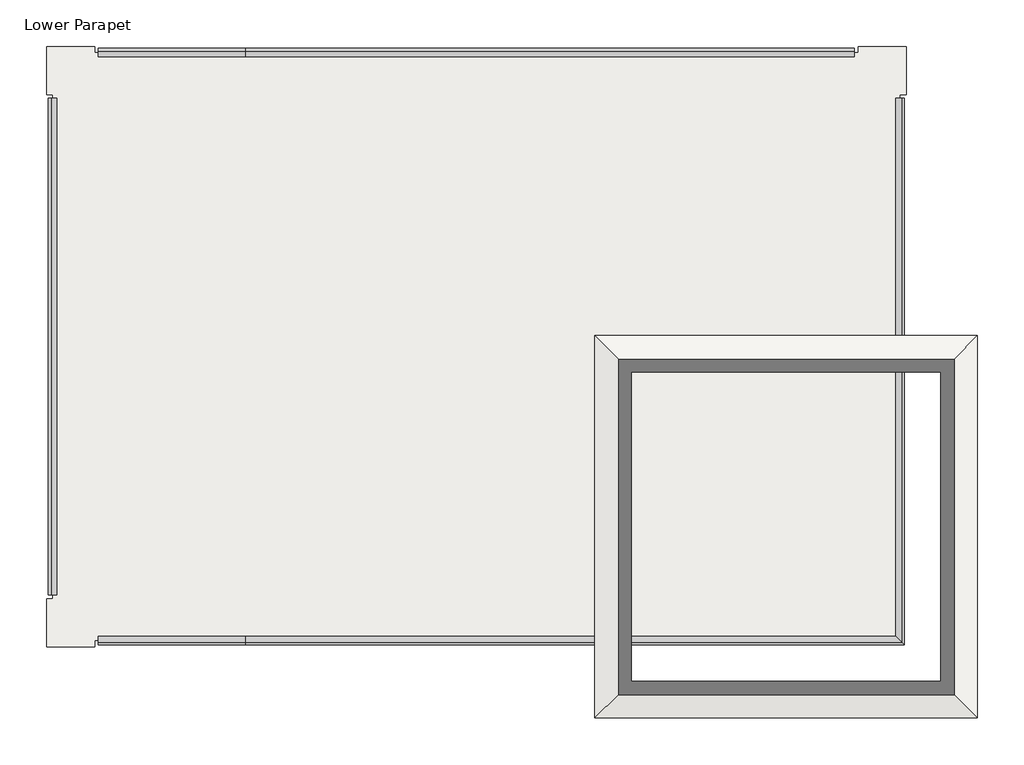
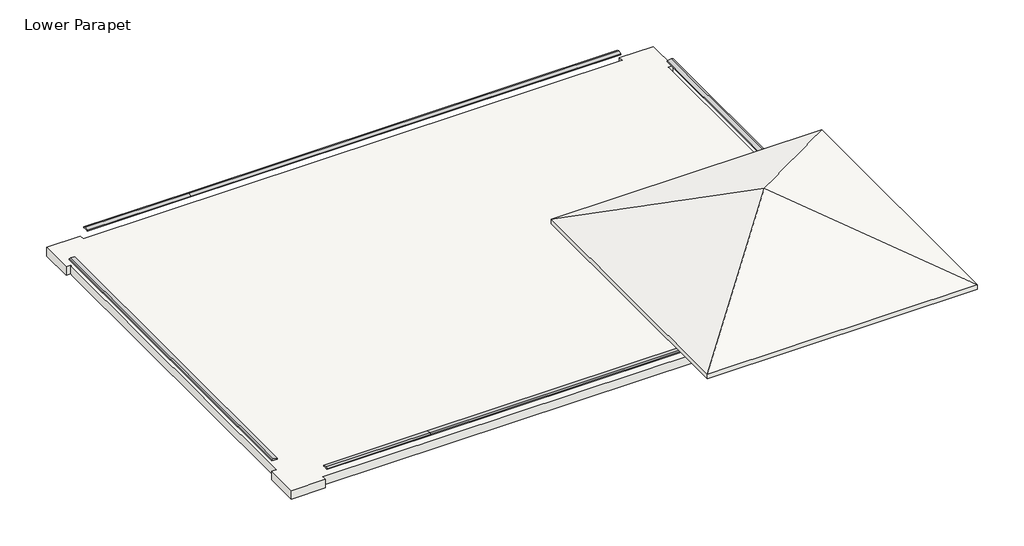
# One storey: 6 proxies, 2 roofs.
"""IFC4 building model written with IfcOpenShell, lengths in millimetres."""

import ifcopenshell
import ifcopenshell.guid

model = None  # the IFC model being written
_history = None  # IfcOwnerHistory: only IFC2X3 demands one
_inside = {}  # id of a spatial element -> (the spatial element, [elements in it])
_under = {}  # id of a project, library or spatial element -> (it, [spatial elements below it])
_declared = {}  # id of a project -> (the project, [libraries it declares])
_typed = {}  # id of a type object -> (the type object, [elements of that type])
_made_of = {}  # id of a material, layer set ... -> (it, [elements and type objects made of it])


def new_model(schema):
    """Start an empty IFC model of exactly this schema.

    Asked for "IFC4X3", IfcOpenShell would pick the latest addendum, in which some entities
    have other attributes; the version numbers below select the first issue.
    IFC2X3 requires an IfcOwnerHistory on every rooted entity: one is made here for all.
    """
    global model, _history
    if schema == "IFC4X3":
        model = ifcopenshell.file(schema_version=(4, 3, 0, 0))
    else:
        model = ifcopenshell.file(schema=schema)
    _inside.clear()
    _under.clear()
    _declared.clear()
    _typed.clear()
    _made_of.clear()
    _history = None
    if model.schema == "IFC2X3":
        org = make("IfcOrganization", Name="unknown")
        user = make(
            "IfcPersonAndOrganization",
            ThePerson=make("IfcPerson", FamilyName="unknown"),
            TheOrganization=org,
        )
        app = make(
            "IfcApplication",
            ApplicationDeveloper=org,
            Version="unknown",
            ApplicationFullName="unknown",
            ApplicationIdentifier="unknown",
        )
        _history = make(
            "IfcOwnerHistory",
            OwningUser=user,
            OwningApplication=app,
            ChangeAction="ADDED",
            CreationDate=0,
        )
    return model


def make(cls, **values):
    """One entity of the class cls with the attributes given. An attribute that is None is left unset."""
    return model.create_entity(
        cls, **{name: value for name, value in values.items() if value is not None}
    )


def rooted(cls, **values):
    """An entity with a GlobalId (a new one), such as an element, a storey or a relation."""
    return make(cls, GlobalId=ifcopenshell.guid.new(), OwnerHistory=_history, **values)


def si_unit(unit_type, name, prefix=None):
    """IfcSIUnit, for example si_unit("LENGTHUNIT", "METRE", prefix="MILLI")."""
    return make("IfcSIUnit", UnitType=unit_type, Prefix=prefix, Name=name)


def assignment(units):
    """IfcUnitAssignment: the units of a project."""
    return None if units is None else make("IfcUnitAssignment", Units=units)


def point(xyz):
    """IfcCartesianPoint."""
    return None if xyz is None else make("IfcCartesianPoint", Coordinates=xyz)


def direction(xyz):
    """IfcDirection."""
    return None if xyz is None else make("IfcDirection", DirectionRatios=xyz)


def frame(location, z_axis=None, x_axis=None):
    """IfcAxis2Placement3D, a coordinate frame: its origin and axes. An axis left out is left unset."""
    return make(
        "IfcAxis2Placement3D",
        Location=point(location),
        Axis=direction(z_axis),
        RefDirection=direction(x_axis),
    )


def origin():
    """The frame at (0, 0, 0) with its axes left unset."""
    return frame((0.0, 0.0, 0.0))


def place(relative_to, where):
    """IfcLocalPlacement: puts the frame where relative to a parent placement (None: the world)."""
    return make(
        "IfcLocalPlacement", PlacementRelTo=relative_to, RelativePlacement=where
    )


def context(
    kind, dimensions, precision=None, world=None, true_north=None, identifier=None
):
    """IfcGeometricRepresentationContext, for example the 3D "Model" context."""
    return make(
        "IfcGeometricRepresentationContext",
        ContextIdentifier=identifier,
        ContextType=kind,
        CoordinateSpaceDimension=dimensions,
        Precision=precision,
        WorldCoordinateSystem=world,
        TrueNorth=true_north,
    )


def project(units=None, contexts=None):
    """IfcProject with its units and contexts."""
    return rooted(
        "IfcProject",
        Name="project",
        RepresentationContexts=contexts,
        UnitsInContext=assignment(units),
    )


def spatial(cls, under=None, at=None, **own):
    """A site, building, storey or space (cls), placed at a placement, below another one or the project."""
    s = rooted(cls, ObjectPlacement=at, **own)
    if under is not None:
        _under.setdefault(under.id(), (under, []))[1].append(s)
    return s


def faces_of(points, faces, orient=None, outer=None):
    """IfcFace entities. A face is a list of loops; a loop is a list of indices into points, from 0.

    orient and outer hold one flag for each loop. By default every Orientation is true, the
    first loop of a face is its IfcFaceOuterBound and the others are IfcFaceBound.
    """
    made = []
    for i, loops in enumerate(faces):
        bounds = []
        for j, loop in enumerate(loops):
            is_outer = j == 0 if outer is None else outer[i][j]
            bounds.append(
                make(
                    "IfcFaceOuterBound" if is_outer else "IfcFaceBound",
                    Bound=make("IfcPolyLoop", Polygon=[points[k] for k in loop]),
                    Orientation=True if orient is None else orient[i][j],
                )
            )
        made.append(make("IfcFace", Bounds=bounds))
    return made


def faceted_brep(points, faces, orient=None, outer=None, voids=None):
    """IfcFacetedBrep: a solid bounded by flat faces; with voids (closed shells), ...WithVoids."""
    shared = [point(p) for p in points]
    hull = make("IfcClosedShell", CfsFaces=faces_of(shared, faces, orient, outer))
    if voids is None:
        return make("IfcFacetedBrep", Outer=hull)
    return make(
        "IfcFacetedBrepWithVoids",
        Outer=hull,
        Voids=[
            make(cls, CfsFaces=faces_of(shared, fs, o, b)) for cls, fs, o, b in voids
        ],
    )


def shape(context_of_items, identifier, shape_type, items):
    """IfcShapeRepresentation: the items that make up one representation, for example the "Body"."""
    return make(
        "IfcShapeRepresentation",
        ContextOfItems=context_of_items,
        RepresentationIdentifier=identifier,
        RepresentationType=shape_type,
        Items=items,
    )


def made_of(thing, what):
    """Note that an element or type object is made of a material, layer set ...; save() writes the relation."""
    if what is not None:
        _made_of.setdefault(what.id(), (what, []))[1].append(thing)
    return thing


def element(
    cls,
    number,
    at=None,
    inside=None,
    cuts=None,
    type_object=None,
    material=None,
    context=None,
    identifier="Body",
    shape_type=None,
    held_by="IfcProductDefinitionShape",
    body=None,
    shapes=None,
    **own,
):
    """One element of the class cls, such as IfcWall. Its Tag is "e" and its number.

    at: its placement. inside: the storey or other place that contains it. cuts: it is an
    opening in that element (IfcRelVoidsElement). A single representation is given by context,
    identifier, shape_type and body (its items); several are given by shapes. held_by: the class
    of the entity that holds the representations. save() writes the other relations.
    """
    e = rooted(cls, Tag="e%d" % number, ObjectPlacement=at, **own)
    if body is not None:
        shapes = [shape(context, identifier, shape_type, body)]
    if shapes is not None:
        e.Representation = make(held_by, Representations=shapes)
    if inside is not None:
        _inside.setdefault(inside.id(), (inside, []))[1].append(e)
    if cuts is not None:
        rooted(
            "IfcRelVoidsElement", RelatingBuildingElement=cuts, RelatedOpeningElement=e
        )
    if type_object is not None:
        _typed.setdefault(type_object.id(), (type_object, []))[1].append(e)
    return made_of(e, material)


def aggregate(whole, parts):
    """IfcRelAggregates: a whole, such as a stair, and the parts it consists of."""
    return rooted("IfcRelAggregates", RelatingObject=whole, RelatedObjects=parts)


def save(model, path):
    """Write the relations noted so far, then the file.

    IfcRelAggregates (storeys below a building ...), IfcRelContainedInSpatialStructure (elements
    in a storey), IfcRelDefinesByType, IfcRelAssociatesMaterial and IfcRelDeclares: one each for
    every whole, place, type object, material and project.
    """
    for whole, parts in _under.values():
        aggregate(whole, parts)
    for where, things in _inside.values():
        rooted(
            "IfcRelContainedInSpatialStructure",
            RelatedElements=things,
            RelatingStructure=where,
        )
    for kind, things in _typed.values():
        rooted("IfcRelDefinesByType", RelatedObjects=things, RelatingType=kind)
    for what, things in _made_of.values():
        rooted("IfcRelAssociatesMaterial", RelatedObjects=things, RelatingMaterial=what)
    for by, libraries in _declared.values():
        rooted("IfcRelDeclares", RelatingContext=by, RelatedDefinitions=libraries)
    model.write(path)


model = new_model("IFC4")

# Units and contexts
model_context = context("Model", 3, world=origin())
ifc_project = project(units=[si_unit("LENGTHUNIT", "METRE", prefix="MILLI")], contexts=[model_context])

# Site, building, storey
site = spatial("IfcSite", under=ifc_project)
building = spatial("IfcBuilding", under=site)
storey = spatial("IfcBuildingStorey", under=building, Name="Lower Parapet", Elevation=7620.0)

# Proxies
placement = place(None, origin())
element("IfcBuildingElementProxy", 1, Name="Wall Sweeps", at=placement, inside=storey, context=model_context, shape_type="Brep", body=[
    faceted_brep([(-20031.8727721, 13964.8686943, 7683.5), (-20031.8727721, 14244.2686943, 7721.6), (-20031.8727721, 14371.2686943, 7683.5), (-20031.8727721, 14371.2686943, 7620.0), (-20031.8727721, 14345.8686943, 7620.0), (-20031.8727721, 13993.4436943, 7620.0), (-20031.8727721, 13964.8686943, 7620.0), (-12953.2102721, 13964.8686943, 7683.5), (-12953.2102721, 13964.8686943, 7620.0), (-12953.2102721, 13993.4436943, 7620.0), (-12953.2102721, 14345.8686943, 7620.0), (-12953.2102721, 14371.2686943, 7620.0), (-12953.2102721, 14371.2686943, 7683.5), (-12953.2102721, 14244.2686943, 7721.6)], [[[0, 1, 2, 3, 4, 5, 6]], [[7, 8, 9, 10, 11, 12, 13]], [[1, 0, 7, 13]], [[2, 1, 13, 12]], [[3, 2, 12, 11]], [[6, 5, 4, 3, 11, 10, 9, 8]], [[0, 6, 8, 7]]]),
])
element("IfcBuildingElementProxy", 2, Name="Wall Sweeps", at=placement, inside=storey, context=model_context, shape_type="Brep", body=[
    faceted_brep([(18449.1272279, 11958.2686943, 7683.5), (18728.5272279, 11958.2686943, 7721.6), (18855.5272279, 11958.2686943, 7683.5), (18855.5272279, 11958.2686943, 7620.0), (18830.1272279, 11958.2686943, 7620.0), (18477.7022279, 11958.2686943, 7620.0), (18449.1272279, 11958.2686943, 7620.0), (18449.1272279, -14025.9313057, 7683.5), (18449.1272279, -14025.9313057, 7620.0), (18855.5272279, -14432.3313057, 7620.0), (18855.5272279, -14432.3313057, 7683.5), (18728.5272279, -14305.3313057, 7721.6)], [[[0, 1, 2, 3, 4, 5, 6]], [[7, 8, 9, 10, 11]], [[1, 0, 7, 11]], [[2, 1, 11, 10]], [[3, 2, 10, 9]], [[6, 5, 4, 3, 9, 8]], [[0, 6, 8, 7]]]),
])
element("IfcBuildingElementProxy", 3, Name="Wall Sweeps", at=placement, inside=storey, context=model_context, shape_type="Brep", body=[
    faceted_brep([(18449.1272279, -14025.9313057, 7683.5), (18728.5272279, -14305.3313057, 7721.6), (18855.5272279, -14432.3313057, 7683.5), (18855.5272279, -14432.3313057, 7620.0), (18449.1272279, -14025.9313057, 7620.0), (-12953.2102721, -14025.9313057, 7683.5), (-12953.2102721, -14025.9313057, 7620.0), (-12953.2102721, -14054.5063057, 7620.0), (-12953.2102721, -14406.9313057, 7620.0), (-12953.2102721, -14432.3313057, 7620.0), (-12953.2102721, -14432.3313057, 7683.5), (-12953.2102721, -14305.3313057, 7721.6)], [[[0, 1, 2, 3, 4]], [[5, 6, 7, 8, 9, 10, 11]], [[1, 0, 5, 11]], [[2, 1, 11, 10]], [[3, 2, 10, 9]], [[4, 3, 9, 8, 7, 6]], [[0, 4, 6, 5]]]),
])
element("IfcBuildingElementProxy", 4, Name="Wall Sweeps", at=placement, inside=storey, context=model_context, shape_type="Brep", body=[
    faceted_brep([(-12953.2102721, 13964.8686943, 7683.5), (-12953.2102721, 14244.2686943, 7721.6), (-12953.2102721, 14371.2686943, 7683.5), (-12953.2102721, 14371.2686943, 7620.0), (-12953.2102721, 14345.8686943, 7620.0), (-12953.2102721, 13993.4436943, 7620.0), (-12953.2102721, 13964.8686943, 7620.0), (16442.5272279, 13964.8686943, 7683.5), (16442.5272279, 13964.8686943, 7620.0), (16442.5272279, 13993.4436943, 7620.0), (16442.5272279, 14345.8686943, 7620.0), (16442.5272279, 14371.2686943, 7620.0), (16442.5272279, 14371.2686943, 7683.5), (16442.5272279, 14244.2686943, 7721.6)], [[[0, 1, 2, 3, 4, 5, 6]], [[7, 8, 9, 10, 11, 12, 13]], [[1, 0, 7, 13]], [[2, 1, 13, 12]], [[3, 2, 12, 11]], [[6, 5, 4, 3, 11, 10, 9, 8]], [[0, 6, 8, 7]]]),
])
element("IfcBuildingElementProxy", 5, Name="Wall Sweeps", at=placement, inside=storey, context=model_context, shape_type="Brep", body=[
    faceted_brep([(-12953.2102721, -14025.9313057, 7683.5), (-12953.2102721, -14305.3313057, 7721.6), (-12953.2102721, -14432.3313057, 7683.5), (-12953.2102721, -14432.3313057, 7620.0), (-12953.2102721, -14406.9313057, 7620.0), (-12953.2102721, -14054.5063057, 7620.0), (-12953.2102721, -14025.9313057, 7620.0), (-20031.8727721, -14025.9313057, 7683.5), (-20031.8727721, -14025.9313057, 7620.0), (-20031.8727721, -14054.5063057, 7620.0), (-20031.8727721, -14406.9313057, 7620.0), (-20031.8727721, -14432.3313057, 7620.0), (-20031.8727721, -14432.3313057, 7683.5), (-20031.8727721, -14305.3313057, 7721.6)], [[[0, 1, 2, 3, 4, 5, 6]], [[7, 8, 9, 10, 11, 12, 13]], [[1, 0, 7, 13]], [[2, 1, 13, 12]], [[3, 2, 12, 11]], [[6, 5, 4, 3, 11, 10, 9, 8]], [[0, 6, 8, 7]]]),
])
element("IfcBuildingElementProxy", 6, Name="Wall Sweeps", at=placement, inside=storey, context=model_context, shape_type="Brep", body=[
    faceted_brep([(-22038.4727721, -12019.3313057, 7683.5), (-22317.8727721, -12019.3313057, 7721.6), (-22444.8727721, -12019.3313057, 7683.5), (-22444.8727721, -12019.3313057, 7620.0), (-22419.4727721, -12019.3313057, 7620.0), (-22067.0477721, -12019.3313057, 7620.0), (-22038.4727721, -12019.3313057, 7620.0), (-22038.4727721, 11958.2686943, 7683.5), (-22038.4727721, 11958.2686943, 7620.0), (-22067.0477721, 11958.2686943, 7620.0), (-22419.4727721, 11958.2686943, 7620.0), (-22444.8727721, 11958.2686943, 7620.0), (-22444.8727721, 11958.2686943, 7683.5), (-22317.8727721, 11958.2686943, 7721.6)], [[[0, 1, 2, 3, 4, 5, 6]], [[7, 8, 9, 10, 11, 12, 13]], [[1, 0, 7, 13]], [[2, 1, 13, 12]], [[3, 2, 12, 11]], [[6, 5, 4, 3, 11, 10, 9, 8]], [[0, 6, 8, 7]]]),
])

# Roofs
element("IfcRoof", 7, ObjectType="Bar Joist Flat Roof", at=placement, inside=storey, context=model_context, shape_type="Brep", body=[
    faceted_brep([(18642.8022279, 12145.5936943, 6400.8), (18642.8022279, -14219.6063057, 6400.8), (-20219.1977721, -14219.6063057, 6400.8), (-20219.1977721, -14524.4063057, 6400.8), (-22536.9477721, -14524.4063057, 6400.8), (-22536.9477721, -12206.6563057, 6400.8), (-22232.1477721, -12206.6563057, 6400.8), (-22232.1477721, -12019.3313057, 6400.8), (-22232.1477721, 11958.2686943, 6400.8), (-22232.1477721, 12145.5936943, 6400.8), (-22536.9477721, 12145.5936943, 6400.8), (-22536.9477721, 14463.3436943, 6400.8), (-20219.1977721, 14463.3436943, 6400.8), (-20219.1977721, 14158.5436943, 6400.8), (16629.8522279, 14158.5436943, 6400.8), (16629.8522279, 14463.3436943, 6400.8), (18947.6022279, 14463.3436943, 6400.8), (18947.6022279, 12145.5936943, 6400.8), (18642.8022279, -14219.6063057, 7016.75), (18642.8022279, 12145.5936943, 7016.75), (18947.6022279, 12145.5936943, 7016.75), (18947.6022279, 14463.3436943, 7016.75), (16629.8522279, 14463.3436943, 7016.75), (16629.8522279, 14158.5436943, 7016.75), (-20219.1977721, 14158.5436943, 7016.75), (-20219.1977721, 14463.3436943, 7016.75), (-22536.9477721, 14463.3436943, 7016.75), (-22536.9477721, 12145.5936943, 7016.75), (-22232.1477721, 12145.5936943, 7016.75), (-22232.1477721, 11958.2686943, 7016.75), (-22232.1477721, -12019.3313057, 7016.75), (-22232.1477721, -12206.6563057, 7016.75), (-22536.9477721, -12206.6563057, 7016.75), (-22536.9477721, -14524.4063057, 7016.75), (-20219.1977721, -14524.4063057, 7016.75), (-20219.1977721, -14219.6063057, 7016.75)], [[[0, 1, 2, 3, 4, 5, 6, 7, 8, 9, 10, 11, 12, 13, 14, 15, 16, 17]], [[18, 19, 20, 21, 22, 23, 24, 25, 26, 27, 28, 29, 30, 31, 32, 33, 34, 35]], [[19, 18, 1, 0]], [[24, 23, 14, 13]], [[31, 30, 29, 28, 9, 8, 7, 6]], [[18, 35, 2, 1]], [[23, 22, 15, 14]], [[22, 21, 16, 15]], [[25, 24, 13, 12]], [[26, 25, 12, 11]], [[27, 26, 11, 10]], [[28, 27, 10, 9]], [[32, 31, 6, 5]], [[34, 33, 4, 3]], [[35, 34, 3, 2]], [[33, 32, 5, 4]], [[21, 20, 17, 16]], [[20, 19, 0, 17]]]),
])
element("IfcRoof", 8, ObjectType="Canopy Roof", at=placement, inside=storey, context=model_context, shape_type="Brep", body=[
    faceted_brep([(13154.0209779, -8730.8250557, 12540.853125), (22386.1272279, 501.2811943, 7924.8), (22386.1272279, -17962.9313057, 7924.8), (3921.9147279, 501.2811943, 7924.8), (3921.9147279, -17962.9313057, 7924.8), (22386.1272279, 501.2811943, 8258.4772439), (13154.0209779, -8730.8250557, 12874.5303689), (22386.1272279, -17962.9313057, 8258.4772439), (3921.9147279, 501.2811943, 8258.4772439), (3921.9147279, -17962.9313057, 8258.4772439)], [[[0, 1, 2]], [[3, 0, 4]], [[1, 0, 3]], [[4, 0, 2]], [[5, 6, 7]], [[8, 9, 6]], [[5, 8, 6]], [[9, 7, 6]], [[3, 8, 5, 1]], [[4, 9, 8, 3]], [[2, 7, 9, 4]], [[1, 5, 7, 2]]]),
])

save(model, "model.ifc")

# Revit data of these elements
# Type "Bar Joist Flat Roof"
#   Assembly Code = "B1020"
#   Layers, outside or top first: 6.35 mm "Roofing - EPDM Membrane" (function 4); 76.2 mm "Insulation / Thermal Barriers - Rigid insulation" (function 3); 76.2 mm "Metal - Steel" (function 1); 457.2 mm "Structure - Steel Bar Joist Layer" (function 1)
# Type "Canopy Roof"
#   Assembly Code = "B1020"
#   Layers, outside or top first: 12.7 mm "Roofing - Metal Standing Seam" (function 4); 0 mm "Roofing - EPDM Membrane" (function 100); 19.05 mm "Wood - Sheathing - plywood" (function 2); 266.7 mm "Metal - Stud Layer" (function 1)
# Elements 1, 2, 3, 4, 5, 6 (IfcBuildingElementProxy)
#   Phase Created = New Construction
#   Materials on its faces: "Precast Cap"
# Element 7 (IfcRoof, "Bar Joist Flat Roof")
#   built-in parameter 1001705 = 23.0208 (stored number, unit not read)
#   built-in parameter 1001701 = -4 (stored number, unit not read)
#   built-in parameter 1001710 = 33615
#   Phase Created = New Construction
#   Materials on its faces: "Structure - Steel Bar Joist Layer", "Roofing - EPDM Membrane"
# Element 8 (IfcRoof, "Canopy Roof")
#   built-in parameter 1001705 = 42.2393 (stored number, unit not read)
#   built-in parameter 1001701 = 1 (stored number, unit not read)
#   built-in parameter 1001710 = 33615
#   Phase Created = New Construction
#   Materials on its faces: "Roofing - Metal Standing Seam", "Metal - Stud Layer"
# Materials
#   "Roofing - EPDM Membrane": class "Plastic", colour RGB 127 127 127, transparency 0, Description = "Exterior finish, roofing", Cost = 0
#   "Insulation / Thermal Barriers - Rigid insulation": class "Miscellaneous", colour RGB 127 127 127, transparency 0, Cost = 0
#   "Metal - Steel": class "Metal", colour RGB 199 199 199, transparency 0, Cost = 0
#   "Structure - Steel Bar Joist Layer": class "Metal", colour RGB 127 127 127, transparency 0, Cost = 0
#   "Roofing - Metal Standing Seam": class "Metal", colour RGB 0 128 64, transparency 0, Description = "Exterior finish, roofing", Cost = 0
#   "Wood - Sheathing - plywood": class "Wood", colour RGB 212 179 113, transparency 0, Cost = 0
#   "Metal - Stud Layer": class "Metal", colour RGB 199 199 199, transparency 0, Cost = 0
#   "Precast Cap": class "Stucco", colour RGB 129 132 118, transparency 0, Cost = 0
